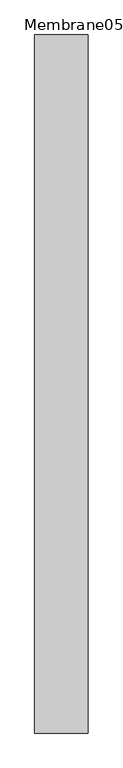
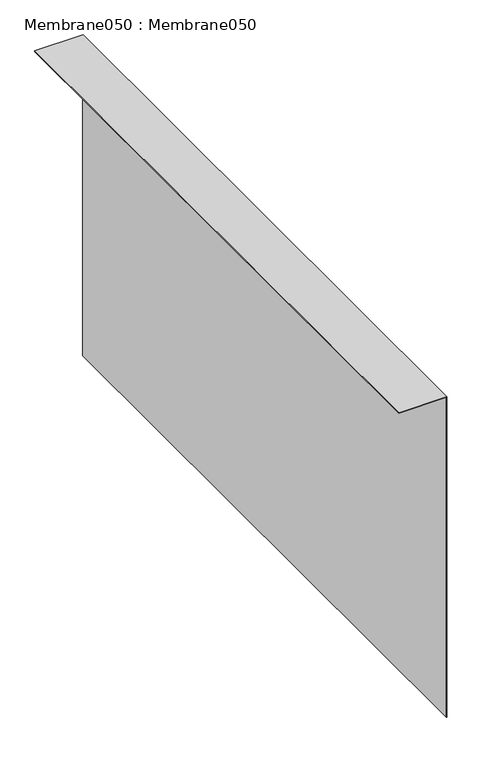
"""IFC4 building model written with IfcOpenShell, lengths in millimetres: proxy geometry, Membrane050 : Membrane050."""

from ifc_helpers import new_model, si_unit, frame, origin, place, context, project, spatial, polyline, outline, extrude, source, transform, mapped, element, save


def membrane050_membrane050_cd8ca409(model_context):
    return source(origin(), model_context, "Body", "SweptSolid", [
        extrude(outline(polyline([(33387.09375, -10092.3525391), (32314.8961275, -10092.3525391), (32314.8961275, -10090.3525391), (33389.09375, -10090.3525391), (33389.09375, -10243.8017578), (33387.09375, -10243.8017578), (33387.09375, -10092.3525391)])), frame((0.0, 7982.1531721, 0.0), z_axis=(0.0, 1.0, 0.0), x_axis=(0.0, 0.0, 1.0)), (0.0, 0.0, 1.0), 2000.0),
    ])


if __name__ == "__main__":
    model = new_model("IFC4")
    model_context = context("Model", 3, world=origin())
    ifc_project = project(units=[si_unit("LENGTHUNIT", "METRE", prefix="MILLI")], contexts=[model_context])
    site = spatial("IfcSite", under=ifc_project)
    building = spatial("IfcBuilding", under=site)
    placement = place(None, origin())
    membrane050_membrane050_shape = membrane050_membrane050_cd8ca409(model_context)
    element("IfcBuildingElementProxy", 1, Name="Membrane050 : Membrane050", ObjectType="Membrane050 : Membrane050", at=placement, inside=building, context=model_context, shape_type="MappedRepresentation", body=[
        mapped(membrane050_membrane050_shape, transform((0.0, 0.0, 0.0), x_axis=(1.0, 0.0, 0.0), y_axis=(0.0, 1.0, 0.0), z_axis=(0.0, 0.0, 1.0))),
    ])
    save(model, "model.ifc")

# Revit data of these elements
# Type "Membrane050 : Membrane050"
#   NameOverride = "Membrane050"
# Element 1 (IfcBuildingElementProxy, "Membrane050 : Membrane050")
#   Materials on its faces: "BITUMINOUS MEMBRANE - TBD"
# Materials
#   "BITUMINOUS MEMBRANE - TBD": class "Unassigned", colour RGB 0 171 31, transparency 0
